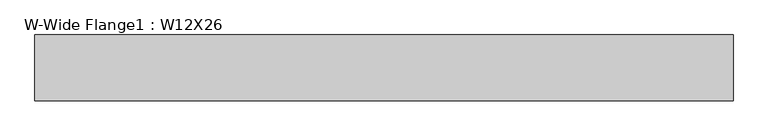
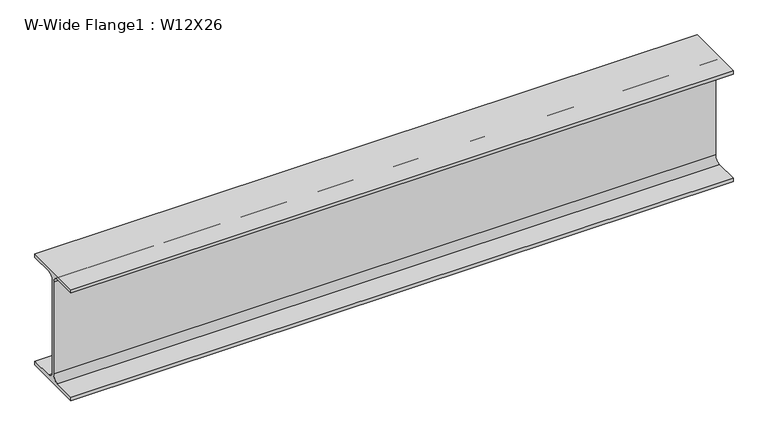
"""IFC4 building model written with IfcOpenShell, lengths in millimetres: beam geometry, W-Wide Flange1 : W12X26."""

from ifc_helpers import new_model, si_unit, point, frame, frame_2d, origin, place, context, project, spatial, polyline, circle_curve, trimmed, segment, composite_curve, outline, extrude, source, transform, mapped, element, save


def w_wide_flange1_w12x26_f9bfccdc(model_context):
    return source(origin(), model_context, "Body", "SweptSolid", [
        extrude(outline(composite_curve([segment(polyline([(82.423, -145.288), (82.423, -154.94), (-82.423, -154.94), (-82.423, -145.288), (-20.2565, -145.288)]), True, "CONTINUOUS"), segment(trimmed(circle_curve(frame_2d((-20.2565, -127.9525)), 17.3355), [point((-20.2565, -145.288))], [point((-2.921, -127.9525))], True, "CARTESIAN"), True, "CONTINUOUS"), segment(polyline([(-2.921, -127.9525), (-2.921, 127.9525)]), True, "CONTINUOUS"), segment(trimmed(circle_curve(frame_2d((-20.2565, 127.9525)), 17.3355), [point((-2.921, 127.9525))], [point((-20.2565, 145.288))], True, "CARTESIAN"), True, "CONTINUOUS"), segment(polyline([(-20.2565, 145.288), (-82.423, 145.288), (-82.423, 154.94), (82.423, 154.94), (82.423, 145.288), (20.2565, 145.288)]), True, "CONTINUOUS"), segment(trimmed(circle_curve(frame_2d((20.2565, 127.9525)), 17.3355), [point((20.2565, 145.288))], [point((2.921, 127.9525))], True, "CARTESIAN"), True, "CONTINUOUS"), segment(polyline([(2.921, 127.9525), (2.921, -127.9525)]), True, "CONTINUOUS"), segment(trimmed(circle_curve(frame_2d((20.2565, -127.9525)), 17.3355), [point((2.921, -127.9525))], [point((20.2565, -145.288))], True, "CARTESIAN"), True, "CONTINUOUS"), segment(polyline([(20.2565, -145.288), (82.423, -145.288)]), True, "CONTINUOUS")], self_intersect=False)), frame((-860.7971936, 0.0, 0.0), z_axis=(1.0, 0.0, 0.0), x_axis=(0.0, 1.0, 0.0)), (0.0, 0.0, 1.0), 1746.6706213),
    ])


if __name__ == "__main__":
    model = new_model("IFC4")
    model_context = context("Model", 3, world=origin())
    ifc_project = project(units=[si_unit("LENGTHUNIT", "METRE", prefix="MILLI")], contexts=[model_context])
    site = spatial("IfcSite", under=ifc_project)
    building = spatial("IfcBuilding", under=site)
    placement = place(None, origin())
    w_wide_flange1_w12x26_shape = w_wide_flange1_w12x26_f9bfccdc(model_context)
    element("IfcBeam", 1, ObjectType="W-Wide Flange1 : W12X26", at=placement, inside=building, context=model_context, shape_type="MappedRepresentation", body=[
        mapped(w_wide_flange1_w12x26_shape, transform((0.0, 0.0, 0.0), x_axis=(1.0, 0.0, 0.0), y_axis=(0.0, 1.0, 0.0), z_axis=(0.0, 0.0, 1.0))),
    ])
    save(model, "model.ifc")

# Revit data of these elements
# Type "W-Wide Flange1 : W12X26"
#   Assembly Code = "B10"
#   W = 26
#   Start Extension Calculation [instance default] = 10' - 0"
#   Start Extension [instance default] = -0' - 0 1/2"
#   End Extension Calculation [instance default] = 10' - 0"
#   End Extension [instance default] = -0' - 0 1/2"
#   Length [instance default] = 5' - 0"
#   bf = 0' - 6.49"
#   d = 1' - 0.2"
#   k = 0' - 1 1/16"
#   k2 = 0' - 0.6825"
#   tf = 0' - 0.38"
#   tw = 0' - 0.23"
#   A = 0.053125 SF
#   Structural Material [instance default] = Metal - Steel - ASTM A992
# Element 1 (IfcBeam, "W-Wide Flange1 : W12X26")
#   Materials on its faces: "Metal - Steel - ASTM A992"
# Materials
#   "Metal - Steel - ASTM A992": class "Metal", colour RGB 199 199 199, transparency 0
